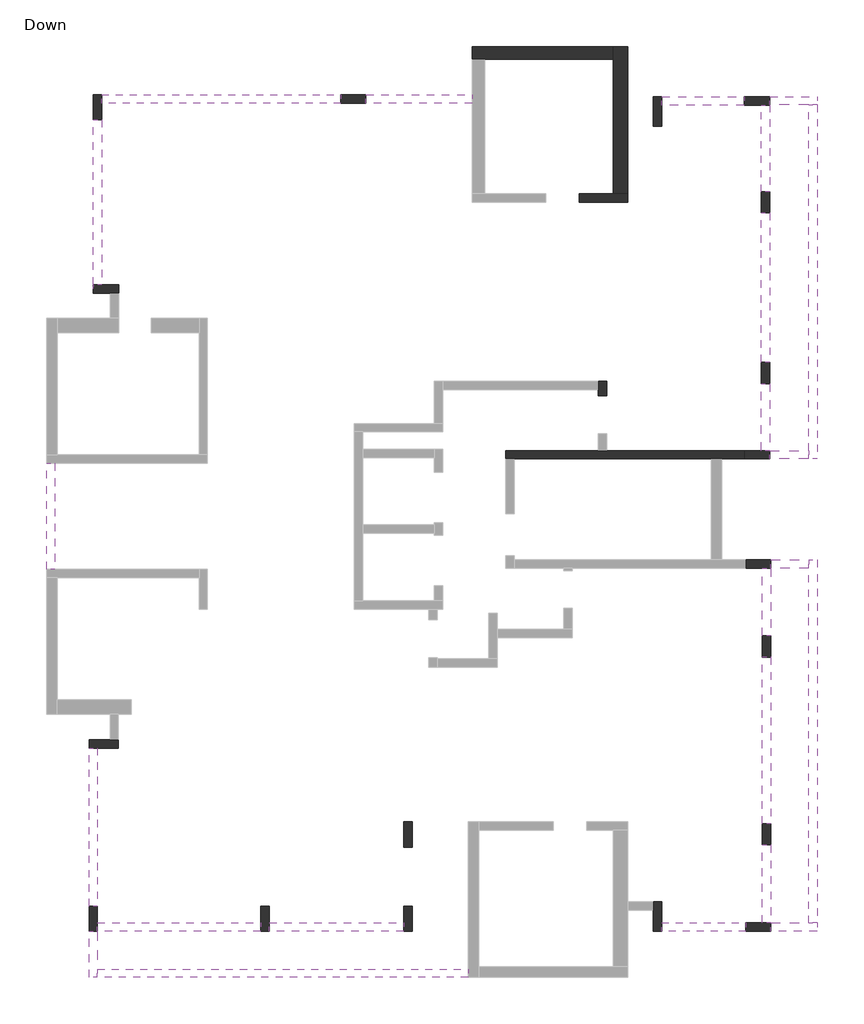
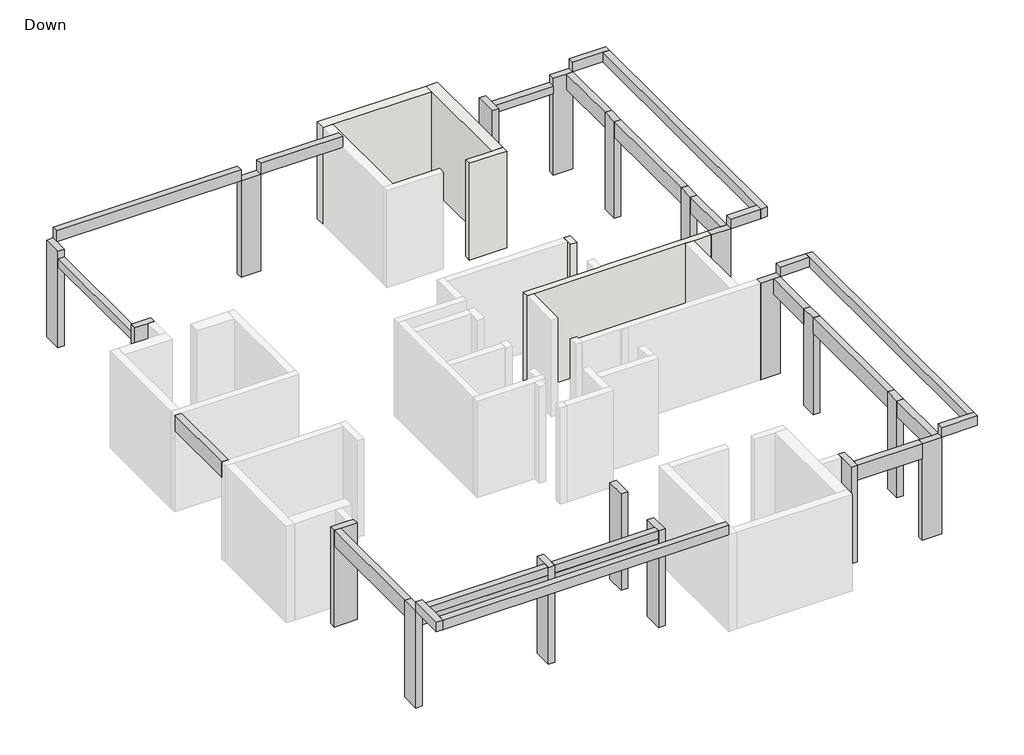
# One storey, part 2 of 2: 23 beams, 18 columns, 5 walls.
"""IFC4 building model written with IfcOpenShell, lengths in millimetres."""

from ifc_helpers import new_model, si_unit, frame, origin, origin_with_axes, place, context, project, spatial, polyline, outline, extrude, faceted_brep, element, save

model = new_model("IFC4")

# Units and contexts
model_context = context("Model", 3, world=origin())
ifc_project = project(units=[si_unit("LENGTHUNIT", "METRE", prefix="MILLI")], contexts=[model_context])

# Site, building, storey
site = spatial("IfcSite", under=ifc_project)
building = spatial("IfcBuilding", under=site)
storey = spatial("IfcBuildingStorey", under=building, Name="Down", Elevation=0.0)

# Beams
placement = place(None, origin())
element("IfcBeam", 1, ObjectType="Concrete Rectengular Beam : 20/50", at=placement, inside=storey, context=model_context, shape_type="Brep", body=[
    faceted_brep([(-11667.5737279, -2465.8036059, 3150.0), (-11467.5737279, -2465.8036059, 3150.0), (-11467.5737279, 47.4292682, 3150.0), (-11667.5737279, 47.4292682, 3150.0), (-11467.5737279, -2465.8036059, 2900.0), (-11467.5737279, -2465.8036059, 2650.0), (-11467.5737279, 47.4292682, 2650.0), (-11467.5737279, 47.4292682, 2900.0), (-11667.5737279, -2465.8036059, 2650.0), (-11667.5737279, 47.4292682, 2650.0)], [[[0, 1, 2, 3]], [[1, 4, 5, 6, 7, 2]], [[5, 8, 9, 6]], [[8, 0, 3, 9]], [[1, 0, 8, 5, 4]], [[3, 2, 7, 6, 9]]]),
])
element("IfcBeam", 2, ObjectType="Concrete Rectengular Beam : 20/50", at=placement, inside=storey, context=model_context, shape_type="Brep", body=[
    faceted_brep([(-10555.9922124, 4197.8205808, 3150.0), (-10555.8228668, 4197.8205808, 3150.0), (-10555.8228668, 4297.8205808, 3150.0), (-10555.9922124, 4297.8205808, 3150.0), (-10355.9922124, 4297.8205808, 2650.0), (-10355.9922124, 8213.0435047, 2650.0), (-10355.9922124, 8213.0435047, 2900.0), (-10355.9922124, 4297.8205808, 2900.0), (-10555.8228668, 4197.8205808, 2650.0), (-10555.9922124, 4197.8205808, 2650.0), (-10555.9922124, 8213.0435047, 2650.0), (-10555.8228668, 4297.8205808, 2650.0), (-10555.9922124, 4297.8205808, 2900.0), (-10555.9922124, 8213.0435047, 2900.0), (-10555.8228668, 4297.8205808, 2900.0)], [[[0, 1, 2, 3]], [[4, 5, 6, 7]], [[8, 9, 10, 5, 4, 11]], [[9, 0, 3, 12, 13, 10]], [[0, 9, 8, 1]], [[11, 4, 7, 14]], [[2, 1, 8, 11, 14]], [[5, 10, 13, 6]], [[12, 14, 7, 6, 13]], [[14, 12, 3, 2]]]),
])
element("IfcBeam", 3, ObjectType="Concrete Rectengular Beam : 20/50", at=placement, inside=storey, context=model_context, shape_type="SweptSolid", body=[
    extrude(outline(polyline([(-1546.8886915, 8813.0435047), (-1546.8886915, 8613.0435047), (-4073.6985753, 8613.0435047), (-4073.6985753, 8813.0435047), (-1546.8886915, 8813.0435047)])), frame((0.0, 0.0, 3150.0), z_axis=(0.0, 0.0, 1.0), x_axis=(1.0, 0.0, 0.0)), (0.0, 0.0, 1.0), 350.0),
])
element("IfcBeam", 4, ObjectType="Concrete Rectengular Beam : 20/50", at=placement, inside=storey, context=model_context, shape_type="SweptSolid", body=[
    extrude(outline(polyline([(2953.3437999, 8567.4646681), (2953.3437999, 8767.4646681), (4922.8790959, 8767.4646681), (4922.8790959, 8567.4646681), (2953.3437999, 8567.4646681)])), frame((0.0, 0.0, 2650.0), z_axis=(0.0, 0.0, 1.0), x_axis=(1.0, 0.0, 0.0)), (0.0, 0.0, 1.0), 250.0),
])
element("IfcBeam", 5, ObjectType="Concrete Rectengular Beam : 20/50", at=placement, inside=storey, context=model_context, shape_type="Brep", body=[
    faceted_brep([(5522.8790959, 8567.4646681, 3150.0), (5322.8790959, 8567.4646681, 3150.0), (5322.8790959, 6503.9942904, 3150.0), (5522.8790959, 6503.9942904, 3150.0), (5522.8790959, 8567.4646681, 2650.0), (5522.8790959, 6503.9942904, 2650.0), (5322.8790959, 8567.4646681, 2650.0), (5322.8790959, 6503.9942904, 2650.0), (5322.8790959, 8567.4646681, 2900.0)], [[[0, 1, 2, 3]], [[4, 0, 3, 5]], [[6, 4, 5, 7]], [[1, 8, 6, 7, 2]], [[1, 0, 4, 6, 8]], [[3, 2, 7, 5]]]),
])
element("IfcBeam", 6, ObjectType="Concrete Rectengular Beam : 20/50", at=placement, inside=storey, context=model_context, shape_type="SweptSolid", body=[
    extrude(outline(polyline([(5322.8790959, 6003.9942904), (5522.8790959, 6003.9942904), (5522.8790959, 2446.2717251), (5322.8790959, 2446.2717251), (5322.8790959, 6003.9942904)])), frame((0.0, 0.0, 2650.0), z_axis=(0.0, 0.0, 1.0), x_axis=(1.0, 0.0, 0.0)), (0.0, 0.0, 1.0), 500.0),
])
element("IfcBeam", 7, ObjectType="Concrete Rectengular Beam : 20/50", at=placement, inside=storey, context=model_context, shape_type="Brep", body=[
    faceted_brep([(5522.8790959, 1946.2717251, 3150.0), (5322.8790959, 1946.2717251, 3150.0), (5322.8790959, 352.3201981, 3150.0), (5522.8790959, 352.3201981, 3150.0), (5322.8790959, 1946.2717251, 2650.0), (5322.8790959, 352.3201981, 2650.0), (5322.8790959, 352.3201981, 2900.0), (5522.8790959, 1946.2717251, 2650.0), (5522.8790959, 352.3201981, 2650.0)], [[[0, 1, 2, 3]], [[1, 4, 5, 6, 2]], [[4, 7, 8, 5]], [[7, 0, 3, 8]], [[1, 0, 7, 4]], [[3, 2, 6, 5, 8]]]),
])
element("IfcBeam", 8, ObjectType="Concrete Rectengular Beam : 20/50", at=placement, inside=storey, context=model_context, shape_type="Brep", body=[
    faceted_brep([(5351.7310336, -4055.4465944, 3150.0), (5551.7310336, -4055.4465944, 3150.0), (5551.7310336, -2446.7479228, 3150.0), (5351.7310336, -2446.7479228, 3150.0), (5351.7310336, -4055.4465944, 2650.0), (5351.7310336, -2446.7479228, 2900.0), (5351.7310336, -2446.7479228, 2650.0), (5551.7310336, -4055.4465944, 2650.0), (5551.7310336, -2446.7479228, 2650.0)], [[[0, 1, 2, 3]], [[4, 0, 3, 5, 6]], [[7, 4, 6, 8]], [[1, 7, 8, 2]], [[1, 0, 4, 7]], [[3, 2, 8, 6, 5]]]),
])
element("IfcBeam", 9, ObjectType="Concrete Rectengular Beam : 20/50", at=placement, inside=storey, context=model_context, shape_type="SweptSolid", body=[
    extrude(outline(polyline([(5551.7310336, -8523.8910533), (5351.7310336, -8523.8910533), (5351.7310336, -4555.4465944), (5551.7310336, -4555.4465944), (5551.7310336, -8523.8910533)])), frame((0.0, 0.0, 2650.0), z_axis=(0.0, 0.0, 1.0), x_axis=(1.0, 0.0, 0.0)), (0.0, 0.0, 1.0), 500.0),
])
element("IfcBeam", 10, ObjectType="Concrete Rectengular Beam : 20/50", at=placement, inside=storey, context=model_context, shape_type="Brep", body=[
    faceted_brep([(5351.7310336, -10874.7377812, 3150.0), (5551.7310336, -10874.7377812, 3150.0), (5551.7310336, -9023.8910533, 3150.0), (5351.7310336, -9023.8910533, 3150.0), (5351.7310336, -10874.7377812, 2650.0), (5351.7310336, -10874.7377812, 2900.0), (5351.7310336, -9023.8910533, 2650.0), (5551.7310336, -10874.7377812, 2650.0), (5551.7310336, -9023.8910533, 2650.0)], [[[0, 1, 2, 3]], [[4, 5, 0, 3, 6]], [[7, 4, 6, 8]], [[1, 7, 8, 2]], [[1, 0, 5, 4, 7]], [[3, 2, 8, 6]]]),
])
element("IfcBeam", 11, ObjectType="Concrete Rectengular Beam : 20/50", at=placement, inside=storey, context=model_context, shape_type="Brep", body=[
    faceted_brep([(2953.3437999, -10874.7377812, 3150.0), (2953.3437999, -11074.7377812, 3150.0), (4951.7310336, -11074.7377812, 3150.0), (4951.7310336, -10874.7377812, 3150.0), (4951.7310336, -10874.7377812, 2900.0), (4951.7310336, -10874.7377812, 2650.0), (2953.3437999, -10874.7377812, 2650.0), (2953.3437999, -10874.7377812, 2900.0), (2953.3437999, -11074.7377812, 2650.0), (4951.7310336, -11074.7377812, 2650.0)], [[[0, 1, 2, 3]], [[0, 3, 4, 5, 6, 7]], [[8, 6, 5, 9]], [[1, 8, 9, 2]], [[1, 0, 7, 6, 8]], [[3, 2, 9, 5, 4]]]),
])
element("IfcBeam", 12, ObjectType="Concrete Rectengular Beam : 20/50", at=placement, inside=storey, context=model_context, shape_type="Brep", body=[
    faceted_brep([(-6576.4457141, -10874.7377812, 3150.0), (-10457.6225223, -10874.7377812, 3150.0), (-10457.6225223, -11073.8349319, 3150.0), (-6576.4457141, -11073.8349319, 3150.0), (-10457.6225223, -10874.7377812, 2650.0), (-10457.6225223, -10874.7377812, 2900.0), (-6576.4457141, -10874.7377812, 2900.0), (-6576.4457141, -10874.7377812, 2650.0), (-10457.6225223, -11074.7377812, 2650.0), (-6576.4457141, -11074.7377812, 2650.0), (-6576.4457141, -11074.7377812, 2900.0), (-10457.6225223, -11074.7377812, 2900.0), (-10457.6225223, -11073.8349319, 2900.0), (-6576.4457141, -11073.8349319, 2900.0)], [[[0, 1, 2, 3]], [[4, 5, 1, 0, 6, 7]], [[8, 4, 7, 9]], [[8, 9, 10, 11]], [[4, 8, 11, 12, 2, 1, 5]], [[9, 7, 6, 0, 3, 13, 10]], [[13, 12, 11, 10]], [[12, 13, 3, 2]]]),
])
element("IfcBeam", 13, ObjectType="Concrete Rectengular Beam : 20/50", at=placement, inside=storey, context=model_context, shape_type="Brep", body=[
    faceted_brep([(-10657.6225223, -10475.5031849, 3150.0), (-10457.6225223, -10475.5031849, 3150.0), (-10457.6225223, -6721.9995493, 3150.0), (-10657.6225223, -6721.9995493, 3150.0), (-10457.6225223, -10475.5031849, 2900.0), (-10457.6225223, -10475.5031849, 2650.0), (-10457.6225223, -6721.9995493, 2650.0), (-10457.6225223, -6721.9995493, 2900.0), (-10657.6225223, -10475.5031849, 2650.0), (-10657.6225223, -6721.9995493, 2650.0)], [[[0, 1, 2, 3]], [[2, 1, 4, 5, 6, 7]], [[5, 8, 9, 6]], [[8, 0, 3, 9]], [[1, 0, 8, 5, 4]], [[3, 2, 7, 6, 9]]]),
])
element("IfcBeam", 14, ObjectType="Concrete Rectengular Beam : 20/50", at=placement, inside=storey, context=model_context, shape_type="Brep", body=[
    faceted_brep([(-3172.9736513, -10874.7377812, 3150.0), (-6376.4457141, -10874.7377812, 3150.0), (-6376.4457141, -11073.8349319, 3150.0), (-3172.9736513, -11073.8349319, 3150.0), (-6376.4457141, -11074.7377812, 2650.0), (-3172.9736513, -11074.7377812, 2650.0), (-3172.9736513, -11074.7377812, 2900.0), (-6376.4457141, -11074.7377812, 2900.0), (-6376.4457141, -10874.7377812, 2650.0), (-3172.9736513, -10874.7377812, 2650.0), (-3172.9736513, -10874.7377812, 2900.0), (-6376.4457141, -10874.7377812, 2900.0), (-6376.4457141, -11073.8349319, 2900.0), (-3172.9736513, -11073.8349319, 2900.0)], [[[0, 1, 2, 3]], [[4, 5, 6, 7]], [[4, 8, 9, 5]], [[1, 0, 10, 9, 8, 11]], [[8, 4, 7, 12, 2, 1, 11]], [[5, 9, 10, 0, 3, 13, 6]], [[13, 12, 7, 6]], [[12, 13, 3, 2]]]),
])
element("IfcBeam", 15, ObjectType="Concrete Rectengular Beam : 20/56", at=placement, inside=storey, context=model_context, shape_type="Brep", body=[
    faceted_brep([(6650.1463257, 8767.4646681, 3460.0), (5522.8790959, 8767.4646681, 3460.0), (5522.8790959, 8567.4646681, 3460.0), (6450.1463257, 8567.4646681, 3460.0), (6650.1463257, 8567.4646681, 3460.0), (5522.8790959, 8567.4646681, 3150.0), (6450.1463257, 8567.4646681, 3150.0), (6650.1463257, 8567.4646681, 3150.0), (6650.1463257, 8767.4646681, 3150.0), (5522.8790959, 8767.4646681, 3150.0)], [[[0, 1, 2, 3, 4]], [[4, 3, 2, 5, 6, 7]], [[1, 0, 8, 9]], [[0, 4, 7, 8]], [[7, 6, 5, 9, 8]], [[2, 1, 9, 5]]]),
])
element("IfcBeam", 16, ObjectType="Concrete Rectengular Beam : 20/56", at=placement, inside=storey, context=model_context, shape_type="Brep", body=[
    faceted_brep([(6650.1463257, 8567.4646681, 3460.0), (6450.1463257, 8567.4646681, 3460.0), (6450.1463257, 352.3201981, 3460.0), (6450.1463257, 152.3201981, 3460.0), (6650.1463257, 152.3201981, 3460.0), (6450.1463257, 8567.4646681, 3150.0), (6450.1463257, 352.3201981, 3150.0), (6450.1463257, 152.3201981, 3150.0), (6650.1463257, 152.3201981, 3150.0), (6650.1463257, 8567.4646681, 3150.0)], [[[0, 1, 2, 3, 4]], [[3, 2, 1, 5, 6, 7]], [[0, 4, 8, 9]], [[1, 0, 9, 5]], [[4, 3, 7, 8]], [[7, 6, 5, 9, 8]]]),
])
element("IfcBeam", 17, ObjectType="Concrete Rectengular Beam : 20/56", at=placement, inside=storey, context=model_context, shape_type="SweptSolid", body=[
    extrude(outline(polyline([(5522.8790959, 152.3201981), (5522.8790959, 352.3201981), (6450.1463257, 352.3201981), (6450.1463257, 152.3201981), (5522.8790959, 152.3201981)])), frame((0.0, 0.0, 3150.0), z_axis=(0.0, 0.0, 1.0), x_axis=(1.0, 0.0, 0.0)), (0.0, 0.0, 1.0), 310.0),
])
element("IfcBeam", 18, ObjectType="Concrete Rectengular Beam : 20/56", at=placement, inside=storey, context=model_context, shape_type="Brep", body=[
    faceted_brep([(-10657.6225223, -11075.5031849, 3460.0), (-10457.6225223, -11075.5031849, 3460.0), (-10457.6225223, -11075.5031849, 3150.0), (-10657.6225223, -11075.5031849, 3150.0), (-10657.6225223, -12173.6155079, 3460.0), (-10457.6225223, -12173.6155079, 3460.0), (-10457.6225223, -11973.6155079, 3460.0), (-10657.6225223, -12173.6155079, 3150.0), (-10457.6225223, -12173.6155079, 3150.0), (-10457.6225223, -11973.6155079, 3150.0)], [[[0, 1, 2, 3]], [[1, 0, 4, 5, 6]], [[4, 0, 3, 7]], [[1, 6, 5, 8, 9, 2]], [[5, 4, 7, 8]], [[3, 2, 9, 8, 7]]]),
])
element("IfcBeam", 19, ObjectType="Concrete Rectengular Beam : 20/56", at=placement, inside=storey, context=model_context, shape_type="SweptSolid", body=[
    extrude(outline(polyline([(-1646.4017034, -11973.6155079), (-1646.4017034, -12173.6155079), (-10457.6225223, -12173.6155079), (-10457.6225223, -11973.6155079), (-1646.4017034, -11973.6155079)])), frame((0.0, 0.0, 3150.0), z_axis=(0.0, 0.0, 1.0), x_axis=(1.0, 0.0, 0.0)), (0.0, 0.0, 1.0), 310.0),
])
element("IfcBeam", 20, ObjectType="Concrete Rectengular Beam : 20/56", at=placement, inside=storey, context=model_context, shape_type="Brep", body=[
    faceted_brep([(5551.7310336, -11074.7377812, 3460.0), (5551.7310336, -10874.7377812, 3460.0), (5551.7310336, -10874.7377812, 3150.0), (5551.7310336, -11074.7377812, 3150.0), (6650.1463257, -11074.7377812, 3460.0), (6650.1463257, -10874.7377812, 3460.0), (6450.1463257, -10874.7377812, 3460.0), (6650.1463257, -11074.7377812, 3150.0), (6650.1463257, -10874.7377812, 3150.0), (6450.1463257, -10874.7377812, 3150.0)], [[[0, 1, 2, 3]], [[1, 0, 4, 5, 6]], [[4, 0, 3, 7]], [[1, 6, 5, 8, 9, 2]], [[5, 4, 7, 8]], [[3, 2, 9, 8, 7]]]),
])
element("IfcBeam", 21, ObjectType="Concrete Rectengular Beam : 20/56", at=placement, inside=storey, context=model_context, shape_type="Brep", body=[
    faceted_brep([(6650.1463257, -2246.7479228, 3460.0), (6450.1463257, -2246.7479228, 3460.0), (6450.1463257, -2446.7479228, 3460.0), (6450.1463257, -10874.7377812, 3460.0), (6650.1463257, -10874.7377812, 3460.0), (6650.1463257, -10874.7377812, 3150.0), (6650.1463257, -2246.7479228, 3150.0), (6450.1463257, -2246.7479228, 3150.0), (6450.1463257, -2446.7479228, 3150.0), (6450.1463257, -10874.7377812, 3150.0)], [[[0, 1, 2, 3, 4]], [[0, 4, 5, 6]], [[3, 2, 1, 7, 8, 9]], [[4, 3, 9, 5]], [[1, 0, 6, 7]], [[6, 5, 9, 8, 7]]]),
])
element("IfcBeam", 22, ObjectType="Concrete Rectengular Beam : 20/56", at=placement, inside=storey, context=model_context, shape_type="SweptSolid", body=[
    extrude(outline(polyline([(5551.7310336, -2446.7479228), (5551.7310336, -2246.7479228), (6450.1463257, -2246.7479228), (6450.1463257, -2446.7479228), (5551.7310336, -2446.7479228)])), frame((0.0, 0.0, 3150.0), z_axis=(0.0, 0.0, 1.0), x_axis=(1.0, 0.0, 0.0)), (0.0, 0.0, 1.0), 310.0),
])
element("IfcBeam", 23, ObjectType="Concrete Rectengular Beam : 20/60", at=placement, inside=storey, context=model_context, shape_type="SweptSolid", body=[
    extrude(outline(polyline([(-10355.9922124, 8613.0435047), (-10355.9922124, 8813.0435047), (-4673.6985753, 8813.0435047), (-4673.6985753, 8613.0435047), (-10355.9922124, 8613.0435047)])), frame((0.0, 0.0, 3150.0), z_axis=(0.0, 0.0, 1.0), x_axis=(1.0, 0.0, 0.0)), (0.0, 0.0, 1.0), 350.0),
])

# Columns
element("IfcColumn", 24, ObjectType="Concrete Rectengular Column : 20/50", at=placement, inside=storey, context=model_context, shape_type="SweptSolid", body=[
    extrude(outline(polyline([(5551.7310336, -8523.8910533), (5551.7310336, -9023.8910533), (5351.7310336, -9023.8910533), (5351.7310336, -8523.8910533), (5551.7310336, -8523.8910533)])), origin_with_axes(), (0.0, 0.0, 1.0), 3150.0),
])
element("IfcColumn", 25, ObjectType="Concrete Rectengular Column : 20/50", at=placement, inside=storey, context=model_context, shape_type="SweptSolid", body=[
    extrude(outline(polyline([(5551.7310336, -4055.4465944), (5551.7310336, -4555.4465944), (5351.7310336, -4555.4465944), (5351.7310336, -4055.4465944), (5551.7310336, -4055.4465944)])), origin_with_axes(), (0.0, 0.0, 1.0), 3150.0),
])
element("IfcColumn", 26, ObjectType="Concrete Rectengular Column : 20/50", at=placement, inside=storey, context=model_context, shape_type="SweptSolid", body=[
    extrude(outline(polyline([(5522.8790959, 6503.9942904), (5522.8790959, 6003.9942904), (5322.8790959, 6003.9942904), (5322.8790959, 6503.9942904), (5522.8790959, 6503.9942904)])), origin_with_axes(), (0.0, 0.0, 1.0), 3150.0),
])
element("IfcColumn", 27, ObjectType="Concrete Rectengular Column : 20/50", at=placement, inside=storey, context=model_context, shape_type="SweptSolid", body=[
    extrude(outline(polyline([(5522.8790959, 2446.2717251), (5522.8790959, 1946.2717251), (5322.8790959, 1946.2717251), (5322.8790959, 2446.2717251), (5522.8790959, 2446.2717251)])), origin_with_axes(), (0.0, 0.0, 1.0), 3150.0),
])
element("IfcColumn", 28, ObjectType="Concrete Rectengular Column : 20/60", at=placement, inside=storey, context=model_context, shape_type="Brep", body=[
    faceted_brep([(-10457.6225223, -10475.5031849, 0.0), (-10457.6225223, -11075.5031849, 0.0), (-10657.6225223, -11075.5031849, 0.0), (-10657.6225223, -10475.5031849, 0.0), (-10457.6225223, -10475.5031849, 3150.0), (-10457.6225223, -10874.7377812, 3150.0), (-10457.6225223, -11073.8349319, 3150.0), (-10457.6225223, -11075.5031849, 3150.0), (-10457.6225223, -11075.5031849, 2900.0), (-10657.6225223, -11075.5031849, 3150.0), (-10657.6225223, -11075.5031849, 2900.0), (-10657.6225223, -10475.5031849, 3150.0)], [[[0, 1, 2, 3]], [[4, 5, 6, 7, 8, 1, 0]], [[7, 9, 10, 2, 1, 8]], [[9, 11, 3, 2, 10]], [[11, 4, 0, 3]], [[4, 11, 9, 7, 6, 5]]]),
])
element("IfcColumn", 29, ObjectType="Concrete Rectengular Column : 20/60", at=placement, inside=storey, context=model_context, shape_type="Brep", body=[
    faceted_brep([(-6376.4457141, -10475.5031849, 0.0), (-6376.4457141, -11075.5031849, 0.0), (-6576.4457141, -11075.5031849, 0.0), (-6576.4457141, -10475.5031849, 0.0), (-6376.4457141, -10475.5031849, 3150.0), (-6376.4457141, -10874.7377812, 3150.0), (-6376.4457141, -11073.8349319, 3150.0), (-6376.4457141, -11075.5031849, 3150.0), (-6376.4457141, -11075.5031849, 2900.0), (-6376.4457141, -10475.5031849, 2900.0), (-6576.4457141, -11075.5031849, 3150.0), (-6576.4457141, -11075.5031849, 2900.0), (-6576.4457141, -11073.8349319, 3150.0), (-6576.4457141, -10874.7377812, 3150.0), (-6576.4457141, -10475.5031849, 3150.0), (-6576.4457141, -10475.5031849, 2900.0)], [[[0, 1, 2, 3]], [[4, 5, 6, 7, 8, 1, 0, 9]], [[7, 10, 11, 2, 1, 8]], [[10, 12, 13, 14, 15, 3, 2, 11]], [[14, 4, 9, 0, 3, 15]], [[4, 14, 13, 12, 10, 7, 6, 5]]]),
])
element("IfcColumn", 30, ObjectType="Concrete Rectengular Column : 20/60", at=placement, inside=storey, context=model_context, shape_type="Brep", body=[
    faceted_brep([(-2972.9736513, -10475.5031849, 0.0), (-2972.9736513, -11075.5031849, 0.0), (-3172.9736513, -11075.5031849, 0.0), (-3172.9736513, -10475.5031849, 0.0), (-2972.9736513, -10475.5031849, 3150.0), (-2972.9736513, -11075.5031849, 3150.0), (-2972.9736513, -11075.5031849, 2900.0), (-3172.9736513, -11075.5031849, 3150.0), (-3172.9736513, -11075.5031849, 2900.0), (-3172.9736513, -11073.8349319, 3150.0), (-3172.9736513, -10874.7377812, 3150.0), (-3172.9736513, -10475.5031849, 3150.0)], [[[0, 1, 2, 3]], [[4, 5, 6, 1, 0]], [[5, 7, 8, 2, 1, 6]], [[7, 9, 10, 11, 3, 2, 8]], [[11, 4, 0, 3]], [[4, 11, 10, 9, 7, 5]]]),
])
element("IfcColumn", 31, ObjectType="Concrete Rectengular Column : 20/60", at=placement, inside=storey, context=model_context, shape_type="Brep", body=[
    faceted_brep([(-2972.9736513, -8473.8910533, 0.0), (-2972.9736513, -9073.8910533, 0.0), (-3172.9736513, -9073.8910533, 0.0), (-3172.9736513, -8473.8910533, 0.0), (-2972.9736513, -8473.8910533, 3150.0), (-2972.9736513, -9073.8910533, 3150.0), (-2972.9736513, -8473.8910533, 2900.0), (-3172.9736513, -9073.8910533, 3150.0), (-3172.9736513, -8473.8910533, 3150.0), (-3172.9736513, -8473.8910533, 2900.0)], [[[0, 1, 2, 3]], [[4, 5, 1, 0, 6]], [[5, 7, 2, 1]], [[7, 8, 9, 3, 2]], [[8, 4, 6, 0, 3, 9]], [[4, 8, 7, 5]]]),
])
element("IfcColumn", 32, ObjectType="Concrete Rectengular Column : 20/60", at=placement, inside=storey, context=model_context, shape_type="Brep", body=[
    faceted_brep([(-10555.8228668, 4297.8205808, 0.0), (-9955.8228668, 4297.8205808, 0.0), (-9955.8228668, 4097.8205808, 0.0), (-10155.8228668, 4097.8205808, 0.0), (-10555.8228668, 4097.8205808, 0.0), (-10555.8228668, 4297.8205808, 3150.0), (-9955.8228668, 4297.8205808, 3150.0), (-9955.8228668, 4297.8205808, 2900.0), (-9955.8228668, 4097.8205808, 3150.0), (-10155.8228668, 4097.8205808, 3150.0), (-10555.8228668, 4097.8205808, 3150.0)], [[[0, 1, 2, 3, 4]], [[5, 6, 7, 1, 0]], [[6, 8, 2, 1, 7]], [[8, 9, 10, 4, 3, 2]], [[10, 5, 0, 4]], [[5, 10, 9, 8, 6]]]),
])
element("IfcColumn", 33, ObjectType="Concrete Rectengular Column : 20/60", at=placement, inside=storey, context=model_context, shape_type="Brep", body=[
    faceted_brep([(-10555.9922124, 8213.0435047, 0.0), (-10555.9922124, 8813.0435047, 0.0), (-10355.9922124, 8813.0435047, 0.0), (-10355.9922124, 8213.0435047, 0.0), (-10555.9922124, 8213.0435047, 3150.0), (-10555.9922124, 8813.0435047, 3150.0), (-10555.9922124, 8213.0435047, 2900.0), (-10355.9922124, 8813.0435047, 3150.0), (-10355.9922124, 8813.0435047, 2900.0), (-10355.9922124, 8213.0435047, 3150.0), (-10355.9922124, 8213.0435047, 2900.0)], [[[0, 1, 2, 3]], [[4, 5, 1, 0, 6]], [[5, 7, 8, 2, 1]], [[7, 9, 10, 3, 2, 8]], [[9, 4, 6, 0, 3, 10]], [[4, 9, 7, 5]]]),
])
element("IfcColumn", 34, ObjectType="Concrete Rectengular Column : 20/60", at=placement, inside=storey, context=model_context, shape_type="Brep", body=[
    faceted_brep([(-4673.6985753, 8813.0435047, 0.0), (-4073.6985753, 8813.0435047, 0.0), (-4073.6985753, 8613.0435047, 0.0), (-4673.6985753, 8613.0435047, 0.0), (-4673.6985753, 8813.0435047, 3150.0), (-4073.6985753, 8813.0435047, 3150.0), (-4073.6985753, 8813.0435047, 2900.0), (-4673.6985753, 8813.0435047, 2900.0), (-4073.6985753, 8613.0435047, 3150.0), (-4073.6985753, 8613.0435047, 2900.0), (-4673.6985753, 8613.0435047, 3150.0), (-4673.6985753, 8613.0435047, 2900.0)], [[[0, 1, 2, 3]], [[4, 5, 6, 1, 0, 7]], [[5, 8, 9, 2, 1, 6]], [[8, 10, 11, 3, 2, 9]], [[10, 4, 7, 0, 3, 11]], [[4, 10, 8, 5]]]),
])
element("IfcColumn", 35, ObjectType="Concrete Rectengular Column : 20/60", at=placement, inside=storey, context=model_context, shape_type="Brep", body=[
    faceted_brep([(4951.7310336, -10874.7377812, 0.0), (5551.7310336, -10874.7377812, 0.0), (5551.7310336, -11074.7377812, 0.0), (4951.7310336, -11074.7377812, 0.0), (4951.7310336, -10874.7377812, 3150.0), (5351.7310336, -10874.7377812, 3150.0), (5551.7310336, -10874.7377812, 3150.0), (5551.7310336, -11074.7377812, 3150.0), (5551.7310336, -11074.7377812, 2900.0), (4951.7310336, -11074.7377812, 3150.0)], [[[0, 1, 2, 3]], [[4, 5, 6, 1, 0]], [[6, 7, 8, 2, 1]], [[7, 9, 3, 2, 8]], [[9, 4, 0, 3]], [[4, 9, 7, 6, 5]]]),
])
element("IfcColumn", 36, ObjectType="Concrete Rectengular Column : 20/60", at=placement, inside=storey, context=model_context, shape_type="Brep", body=[
    faceted_brep([(4951.7310336, -2246.7479228, 0.0), (5551.7310336, -2246.7479228, 0.0), (5551.7310336, -2446.7479228, 0.0), (4951.7310336, -2446.7479228, 0.0), (4951.7310336, -2246.7479228, 3150.0), (5551.7310336, -2246.7479228, 3150.0), (5551.7310336, -2246.7479228, 2900.0), (5551.7310336, -2446.7479228, 3150.0), (5351.7310336, -2446.7479228, 3150.0), (4951.7310336, -2446.7479228, 3150.0)], [[[0, 1, 2, 3]], [[4, 5, 6, 1, 0]], [[5, 7, 2, 1, 6]], [[7, 8, 9, 3, 2]], [[9, 4, 0, 3]], [[4, 9, 8, 7, 5]]]),
])
element("IfcColumn", 37, ObjectType="Concrete Rectengular Column : 20/60", at=placement, inside=storey, context=model_context, shape_type="Brep", body=[
    faceted_brep([(4922.8790959, 8767.4646681, 0.0), (5522.8790959, 8767.4646681, 0.0), (5522.8790959, 8567.4646681, 0.0), (4922.8790959, 8567.4646681, 0.0), (4922.8790959, 8767.4646681, 3150.0), (5522.8790959, 8767.4646681, 3150.0), (5522.8790959, 8767.4646681, 2900.0), (4922.8790959, 8767.4646681, 2900.0), (5522.8790959, 8567.4646681, 3150.0), (5322.8790959, 8567.4646681, 3150.0), (4922.8790959, 8567.4646681, 3150.0), (4922.8790959, 8567.4646681, 2900.0)], [[[0, 1, 2, 3]], [[4, 5, 6, 1, 0, 7]], [[5, 8, 2, 1, 6]], [[8, 9, 10, 11, 3, 2]], [[10, 4, 7, 0, 3, 11]], [[4, 10, 9, 8, 5]]]),
])
element("IfcColumn", 38, ObjectType="Concrete Rectengular Column : 20/60", at=placement, inside=storey, context=model_context, shape_type="Brep", body=[
    faceted_brep([(4922.8790959, 352.3201981, 0.0), (5522.8790959, 352.3201981, 0.0), (5522.8790959, 152.3201981, 0.0), (4922.8790959, 152.3201981, 0.0), (4922.8790959, 352.3201981, 3150.0), (5322.8790959, 352.3201981, 3150.0), (5522.8790959, 352.3201981, 3150.0), (5522.8790959, 152.3201981, 3150.0), (5522.8790959, 152.3201981, 2900.0), (4922.8790959, 152.3201981, 3150.0)], [[[0, 1, 2, 3]], [[4, 5, 6, 1, 0]], [[6, 7, 8, 2, 1]], [[7, 9, 3, 2, 8]], [[9, 4, 0, 3]], [[4, 9, 7, 6, 5]]]),
])
element("IfcColumn", 39, ObjectType="Concrete Rectengular Column : 20/70", at=placement, inside=storey, context=model_context, shape_type="Brep", body=[
    faceted_brep([(-10657.6225223, -6521.9995493, 0.0), (-10157.6225223, -6521.9995493, 0.0), (-9957.6225223, -6521.9995493, 0.0), (-9957.6225223, -6721.9995493, 0.0), (-10657.6225223, -6721.9995493, 0.0), (-10657.6225223, -6521.9995493, 3150.0), (-10157.6225223, -6521.9995493, 3150.0), (-9957.6225223, -6521.9995493, 3150.0), (-9957.6225223, -6721.9995493, 3150.0), (-9957.6225223, -6721.9995493, 2900.0), (-10457.6225223, -6721.9995493, 3150.0), (-10657.6225223, -6721.9995493, 3150.0), (-10657.6225223, -6721.9995493, 2650.0)], [[[0, 1, 2, 3, 4]], [[5, 6, 7, 2, 1, 0]], [[7, 8, 9, 3, 2]], [[8, 10, 11, 12, 4, 3, 9]], [[11, 5, 0, 4, 12]], [[5, 11, 10, 8, 7, 6]]]),
])
element("IfcColumn", 40, ObjectType="Concrete Rectengular Column : 20/70", at=placement, inside=storey, context=model_context, shape_type="Brep", body=[
    faceted_brep([(2953.3437999, -10374.7377812, 0.0), (2953.3437999, -11074.7377812, 0.0), (2753.3437999, -11074.7377812, 0.0), (2753.3437999, -10574.7377812, 0.0), (2753.3437999, -10374.7377812, 0.0), (2953.3437999, -10374.7377812, 3150.0), (2953.3437999, -10874.7377812, 3150.0), (2953.3437999, -11074.7377812, 3150.0), (2953.3437999, -10374.7377812, 2900.0), (2753.3437999, -11074.7377812, 3150.0), (2753.3437999, -10574.7377812, 3150.0), (2753.3437999, -10374.7377812, 3150.0)], [[[0, 1, 2, 3, 4]], [[5, 6, 7, 1, 0, 8]], [[7, 9, 2, 1]], [[9, 10, 11, 4, 3, 2]], [[11, 5, 8, 0, 4]], [[5, 11, 10, 9, 7, 6]]]),
])
element("IfcColumn", 41, ObjectType="Concrete Rectengular Column : 20/70", at=placement, inside=storey, context=model_context, shape_type="Brep", body=[
    faceted_brep([(2953.3437999, 8767.4646681, 0.0), (2953.3437999, 8067.4646681, 0.0), (2753.3437999, 8067.4646681, 0.0), (2753.3437999, 8767.4646681, 0.0), (2953.3437999, 8767.4646681, 3150.0), (2953.3437999, 8067.4646681, 3150.0), (2953.3437999, 8067.4646681, 2900.0), (2953.3437999, 8767.4646681, 2900.0), (2753.3437999, 8067.4646681, 3150.0), (2753.3437999, 8767.4646681, 3150.0)], [[[0, 1, 2, 3]], [[4, 5, 6, 1, 0, 7]], [[5, 8, 2, 1, 6]], [[8, 9, 3, 2]], [[9, 4, 7, 0, 3]], [[4, 9, 8, 5]]]),
])

# Walls
element("IfcWall", 42, ObjectType="20", at=placement, inside=storey, context=model_context, shape_type="Brep", body=[
    faceted_brep([(1452.348775, 2003.8127355, 0.0), (1452.348775, 1803.8127355, 0.0), (1452.348775, 1652.3412467, 0.0), (1452.348775, 1652.3412467, 2900.0), (1452.348775, 1652.3412467, 3150.0), (1452.348775, 1803.8127355, 3150.0), (1452.348775, 2003.8127355, 3150.0), (1652.348775, 2003.8127355, 0.0), (1652.348775, 2003.8127355, 2900.0), (1652.348775, 2003.8127355, 3150.0), (1652.348775, 1652.3412467, 3150.0), (1652.348775, 1652.3412467, 2900.0), (1652.348775, 1652.3412467, 0.0), (1552.348775, 1652.3412467, 3150.0)], [[[0, 1, 2, 3, 4, 5, 6]], [[7, 8, 9, 10, 11, 12]], [[2, 1, 0, 7, 12]], [[4, 3, 2, 12, 11, 10, 13]], [[6, 5, 4, 13, 10, 9]], [[0, 6, 9, 8, 7]]]),
])
element("IfcWall", 43, ObjectType="20", at=placement, inside=storey, context=model_context, shape_type="Brep", body=[
    faceted_brep([(-748.6672985, 152.3201981, 0.0), (-548.6672985, 152.3201981, 0.0), (4133.663356, 152.3201981, 0.0), (4383.663356, 152.3201981, 0.0), (4922.8790959, 152.3201981, 0.0), (4922.8790959, 152.3201981, 3150.0), (4383.663356, 152.3201981, 3150.0), (4133.663356, 152.3201981, 3150.0), (-548.6672985, 152.3201981, 3150.0), (-748.6672985, 152.3201981, 3150.0), (-748.6672985, 352.3201981, 0.0), (-748.6672985, 352.3201981, 2900.0), (-748.6672985, 352.3201981, 3150.0), (1452.348775, 352.3201981, 3150.0), (1652.348775, 352.3201981, 3150.0), (4922.8790959, 352.3201981, 3150.0), (4922.8790959, 352.3201981, 0.0), (1652.348775, 352.3201981, 0.0), (1452.348775, 352.3201981, 0.0)], [[[0, 1, 2, 3, 4, 5, 6, 7, 8, 9]], [[10, 11, 12, 13, 14, 15, 16, 17, 18]], [[4, 3, 2, 1, 0, 10, 18, 17, 16]], [[5, 4, 16, 15]], [[9, 8, 7, 6, 5, 15, 14, 13, 12]], [[0, 9, 12, 11, 10]]]),
])
element("IfcWall", 44, ObjectType="20", at=placement, inside=storey, context=model_context, shape_type="Brep", body=[
    faceted_brep([(1000.2209526, 6257.4646681, 0.0), (2149.9138343, 6257.4646681, 0.0), (2149.9138343, 6257.4646681, 2900.0), (2149.9138343, 6257.4646681, 3150.0), (1000.2209526, 6257.4646681, 3150.0), (1000.2209526, 6257.4646681, 2900.0), (1000.2209526, 6457.4646681, 0.0), (1000.2209526, 6457.4646681, 2900.0), (1000.2209526, 6457.4646681, 3150.0), (1799.9138343, 6457.4646681, 3150.0), (2149.9138343, 6457.4646681, 3150.0), (2149.9138343, 6457.4646681, 0.0), (1799.9138343, 6457.4646681, 0.0)], [[[0, 1, 2, 3, 4, 5]], [[6, 7, 8, 9, 10, 11, 12]], [[1, 0, 6, 12, 11]], [[4, 3, 10, 9, 8]], [[0, 5, 4, 8, 7, 6]], [[3, 2, 1, 11, 10]]]),
])
element("IfcWall", 45, ObjectType="30", at=placement, inside=storey, context=model_context, shape_type="Brep", body=[
    faceted_brep([(1799.9138343, 9957.4646681, 0.0), (-1546.8886915, 9957.4646681, 0.0), (-1546.8886915, 9957.4646681, 3150.0), (1799.9138343, 9957.4646681, 3150.0), (1799.9138343, 9657.4646681, 0.0), (1799.9138343, 9657.4646681, 2900.0), (1799.9138343, 9657.4646681, 3150.0), (-1246.8886915, 9657.4646681, 3150.0), (-1546.8886915, 9657.4646681, 3150.0), (-1546.8886915, 9657.4646681, 0.0), (-1246.8886915, 9657.4646681, 0.0)], [[[0, 1, 2, 3]], [[4, 5, 6, 7, 8, 9, 10]], [[1, 0, 4, 10, 9]], [[3, 2, 8, 7, 6]], [[0, 3, 6, 5, 4]], [[2, 1, 9, 8]]]),
])
element("IfcWall", 46, ObjectType="35", at=placement, inside=storey, context=model_context, shape_type="Brep", body=[
    faceted_brep([(2149.9138343, 6457.4646681, 0.0), (2149.9138343, 9957.4646681, 0.0), (2149.9138343, 9957.4646681, 3150.0), (2149.9138343, 8067.4646681, 3150.0), (2149.9138343, 6457.4646681, 3150.0), (1799.9138343, 6457.4646681, 0.0), (1799.9138343, 6457.4646681, 2900.0), (1799.9138343, 6457.4646681, 3150.0), (1799.9138343, 9657.4646681, 3150.0), (1799.9138343, 9957.4646681, 3150.0), (1799.9138343, 9957.4646681, 0.0), (1799.9138343, 9657.4646681, 0.0)], [[[0, 1, 2, 3, 4]], [[5, 6, 7, 8, 9, 10, 11]], [[1, 0, 5, 11, 10]], [[4, 3, 2, 9, 8, 7]], [[0, 4, 7, 6, 5]], [[2, 1, 10, 9]]]),
])

save(model, "model.ifc")

# Revit data of these elements
# Type "Concrete Rectengular Beam : 20/50"
#   Length [instance default] = 152.4 cm
#   b = 20 cm
#   h = 50 cm
#   Structural Material [instance default] = Concrete
#   Assembly Code = ""
# Type "Concrete Rectengular Beam : 20/56"
#   Length [instance default] = 152.4 cm
#   b = 20 cm
#   h = 56 cm
#   Structural Material [instance default] = Concrete
#   Assembly Code = ""
# Type "Concrete Rectengular Beam : 20/60"
#   Length [instance default] = 152.4 cm
#   b = 20 cm
#   h = 60 cm
#   Structural Material [instance default] = Concrete
#   Assembly Code = ""
# Type "Concrete Rectengular Column : 20/50"
#   b = 20 cm
#   h = 50 cm
#   Structural Material [instance default] = Concrete
# Type "Concrete Rectengular Column : 20/60"
#   b = 20 cm
#   h = 60 cm
#   Structural Material [instance default] = Concrete
# Type "Concrete Rectengular Column : 20/70"
#   b = 20 cm
#   h = 70 cm
#   Structural Material [instance default] = Concrete
# Type "20"
#   Layers, outside or top first: 20 cm "Concrete" (function 1)
# Type "30"
#   Layers, outside or top first: 30 cm "Concrete" (function 1)
# Type "35"
#   Layers, outside or top first: 35 cm "Concrete" (function 1)
# Element 1 (IfcBeam, "Concrete Rectengular Beam : 20/50")
#   Comments = ""
#   Mark = "B2"
#   SOFiSTiK_AMG_Comments = ""
#   SOFiSTiK_AMG_Scheduled = yes
#   SOFiSTiK_AMG_Adjusted = yes
#   Structural Material = Concrete
#   Phase Created = New Construction
#   Materials on its faces: "Concrete"
# Element 2 (IfcBeam, "Concrete Rectengular Beam : 20/50")
#   Comments = ""
#   Mark = "B3"
#   SOFiSTiK_AMG_Comments = ""
#   SOFiSTiK_AMG_Scheduled = yes
#   SOFiSTiK_AMG_Adjusted = yes
#   Structural Material = Concrete
#   Phase Created = New Construction
#   Materials on its faces: "Concrete"
# Element 3 (IfcBeam, "Concrete Rectengular Beam : 20/50")
#   Comments = ""
#   Mark = "B4"
#   SOFiSTiK_AMG_Comments = ""
#   SOFiSTiK_AMG_Scheduled = yes
#   SOFiSTiK_AMG_Adjusted = yes
#   Structural Material = Concrete
#   Phase Created = New Construction
#   Materials on its faces: "Concrete"
# Element 4 (IfcBeam, "Concrete Rectengular Beam : 20/50")
#   Comments = ""
#   Mark = "B5"
#   SOFiSTiK_AMG_Comments = ""
#   SOFiSTiK_AMG_Scheduled = yes
#   SOFiSTiK_AMG_Adjusted = yes
#   Structural Material = Concrete
#   Phase Created = New Construction
#   Materials on its faces: "Concrete"
# Element 5 (IfcBeam, "Concrete Rectengular Beam : 20/50")
#   Comments = ""
#   Mark = "B6"
#   SOFiSTiK_AMG_Comments = ""
#   SOFiSTiK_AMG_Scheduled = yes
#   SOFiSTiK_AMG_Adjusted = yes
#   Structural Material = Concrete
#   Phase Created = New Construction
#   Materials on its faces: "Concrete"
# Element 6 (IfcBeam, "Concrete Rectengular Beam : 20/50")
#   Comments = ""
#   Mark = "B7"
#   SOFiSTiK_AMG_Comments = ""
#   SOFiSTiK_AMG_Scheduled = yes
#   SOFiSTiK_AMG_Adjusted = yes
#   Structural Material = Concrete
#   Phase Created = New Construction
#   Materials on its faces: "Concrete"
# Element 7 (IfcBeam, "Concrete Rectengular Beam : 20/50")
#   Comments = ""
#   Mark = "B8"
#   SOFiSTiK_AMG_Comments = ""
#   SOFiSTiK_AMG_Scheduled = yes
#   SOFiSTiK_AMG_Adjusted = yes
#   Structural Material = Concrete
#   Phase Created = New Construction
#   Materials on its faces: "Concrete"
# Element 8 (IfcBeam, "Concrete Rectengular Beam : 20/50")
#   Comments = ""
#   Mark = "B9"
#   SOFiSTiK_AMG_Comments = ""
#   SOFiSTiK_AMG_Scheduled = yes
#   SOFiSTiK_AMG_Adjusted = yes
#   Structural Material = Concrete
#   Phase Created = New Construction
#   Materials on its faces: "Concrete"
# Element 9 (IfcBeam, "Concrete Rectengular Beam : 20/50")
#   Comments = ""
#   Mark = "B10"
#   SOFiSTiK_AMG_Comments = ""
#   SOFiSTiK_AMG_Scheduled = yes
#   SOFiSTiK_AMG_Adjusted = yes
#   Structural Material = Concrete
#   Phase Created = New Construction
#   Materials on its faces: "Concrete"
# Element 10 (IfcBeam, "Concrete Rectengular Beam : 20/50")
#   Comments = ""
#   Mark = "B11"
#   SOFiSTiK_AMG_Comments = ""
#   SOFiSTiK_AMG_Scheduled = yes
#   SOFiSTiK_AMG_Adjusted = yes
#   Structural Material = Concrete
#   Phase Created = New Construction
#   Materials on its faces: "Concrete"
# Element 11 (IfcBeam, "Concrete Rectengular Beam : 20/50")
#   Comments = ""
#   Mark = "B12"
#   SOFiSTiK_AMG_Comments = ""
#   SOFiSTiK_AMG_Scheduled = yes
#   SOFiSTiK_AMG_Adjusted = yes
#   Structural Material = Concrete
#   Phase Created = New Construction
#   Materials on its faces: "Concrete"
# Element 12 (IfcBeam, "Concrete Rectengular Beam : 20/50")
#   Comments = ""
#   Mark = "B13"
#   SOFiSTiK_AMG_Comments = ""
#   SOFiSTiK_AMG_Scheduled = yes
#   SOFiSTiK_AMG_Adjusted = yes
#   Structural Material = Concrete
#   Phase Created = New Construction
#   Materials on its faces: "Concrete"
# Element 13 (IfcBeam, "Concrete Rectengular Beam : 20/50")
#   Comments = ""
#   Mark = "B14"
#   SOFiSTiK_AMG_Comments = ""
#   SOFiSTiK_AMG_Scheduled = yes
#   SOFiSTiK_AMG_Adjusted = yes
#   Structural Material = Concrete
#   Phase Created = New Construction
#   Materials on its faces: "Concrete"
# Element 14 (IfcBeam, "Concrete Rectengular Beam : 20/50")
#   Comments = ""
#   Mark = "B15"
#   SOFiSTiK_AMG_Comments = ""
#   SOFiSTiK_AMG_Scheduled = yes
#   SOFiSTiK_AMG_Adjusted = yes
#   Structural Material = Concrete
#   Phase Created = New Construction
#   Materials on its faces: "Concrete"
# Element 15 (IfcBeam, "Concrete Rectengular Beam : 20/56")
#   Comments = ""
#   Mark = "B16"
#   SOFiSTiK_AMG_Comments = ""
#   SOFiSTiK_AMG_Scheduled = yes
#   SOFiSTiK_AMG_Adjusted = yes
#   Structural Material = Concrete
#   Phase Created = New Construction
#   Materials on its faces: "Concrete"
# Element 16 (IfcBeam, "Concrete Rectengular Beam : 20/56")
#   Comments = ""
#   Mark = "B17"
#   SOFiSTiK_AMG_Comments = ""
#   SOFiSTiK_AMG_Scheduled = yes
#   SOFiSTiK_AMG_Adjusted = yes
#   Structural Material = Concrete
#   Phase Created = New Construction
#   Materials on its faces: "Concrete"
# Element 17 (IfcBeam, "Concrete Rectengular Beam : 20/56")
#   Comments = ""
#   Mark = "B18"
#   SOFiSTiK_AMG_Comments = ""
#   SOFiSTiK_AMG_Scheduled = yes
#   SOFiSTiK_AMG_Adjusted = yes
#   Structural Material = Concrete
#   Phase Created = New Construction
#   Materials on its faces: "Concrete"
# Element 18 (IfcBeam, "Concrete Rectengular Beam : 20/56")
#   Comments = ""
#   Mark = "B19"
#   SOFiSTiK_AMG_Comments = ""
#   SOFiSTiK_AMG_Scheduled = yes
#   SOFiSTiK_AMG_Adjusted = yes
#   Structural Material = Concrete
#   Phase Created = New Construction
#   Materials on its faces: "Concrete"
# Element 19 (IfcBeam, "Concrete Rectengular Beam : 20/56")
#   Comments = ""
#   Mark = "B20"
#   SOFiSTiK_AMG_Comments = ""
#   SOFiSTiK_AMG_Scheduled = yes
#   SOFiSTiK_AMG_Adjusted = yes
#   Structural Material = Concrete
#   Phase Created = New Construction
#   Materials on its faces: "Concrete"
# Element 20 (IfcBeam, "Concrete Rectengular Beam : 20/56")
#   Comments = ""
#   Mark = "B21"
#   SOFiSTiK_AMG_Comments = ""
#   SOFiSTiK_AMG_Scheduled = yes
#   SOFiSTiK_AMG_Adjusted = yes
#   Structural Material = Concrete
#   Phase Created = New Construction
#   Materials on its faces: "Concrete"
# Element 21 (IfcBeam, "Concrete Rectengular Beam : 20/56")
#   Comments = ""
#   Mark = "B22"
#   SOFiSTiK_AMG_Comments = ""
#   SOFiSTiK_AMG_Scheduled = yes
#   SOFiSTiK_AMG_Adjusted = yes
#   Structural Material = Concrete
#   Phase Created = New Construction
#   Materials on its faces: "Concrete"
# Element 22 (IfcBeam, "Concrete Rectengular Beam : 20/56")
#   Comments = ""
#   Mark = "B23"
#   SOFiSTiK_AMG_Comments = ""
#   SOFiSTiK_AMG_Scheduled = yes
#   SOFiSTiK_AMG_Adjusted = yes
#   Structural Material = Concrete
#   Phase Created = New Construction
#   Materials on its faces: "Concrete"
# Element 23 (IfcBeam, "Concrete Rectengular Beam : 20/60")
#   Comments = ""
#   Mark = "B24"
#   SOFiSTiK_AMG_Comments = ""
#   SOFiSTiK_AMG_Scheduled = yes
#   SOFiSTiK_AMG_Adjusted = yes
#   Structural Material = Concrete
#   Phase Created = New Construction
#   Materials on its faces: "Concrete"
# Element 24 (IfcColumn, "Concrete Rectengular Column : 20/50")
#   Comments = ""
#   Mark = "C1"
#   SOFiSTiK_AMG_Comments = ""
#   SOFiSTiK_AMG_Scheduled = yes
#   SOFiSTiK_AMG_Adjusted = yes
#   Structural Material = Concrete
#   Phase Created = New Construction
#   Materials on its faces: "Concrete"
# Element 25 (IfcColumn, "Concrete Rectengular Column : 20/50")
#   Comments = ""
#   Mark = "C2"
#   SOFiSTiK_AMG_Comments = ""
#   SOFiSTiK_AMG_Scheduled = yes
#   SOFiSTiK_AMG_Adjusted = yes
#   Structural Material = Concrete
#   Phase Created = New Construction
#   Materials on its faces: "Concrete"
# Element 26 (IfcColumn, "Concrete Rectengular Column : 20/50")
#   Comments = ""
#   Mark = "C3"
#   SOFiSTiK_AMG_Comments = ""
#   SOFiSTiK_AMG_Scheduled = yes
#   SOFiSTiK_AMG_Adjusted = yes
#   Structural Material = Concrete
#   Phase Created = New Construction
#   Materials on its faces: "Concrete"
# Element 27 (IfcColumn, "Concrete Rectengular Column : 20/50")
#   Comments = ""
#   Mark = "C4"
#   SOFiSTiK_AMG_Comments = ""
#   SOFiSTiK_AMG_Scheduled = yes
#   SOFiSTiK_AMG_Adjusted = yes
#   Structural Material = Concrete
#   Phase Created = New Construction
#   Materials on its faces: "Concrete"
# Element 28 (IfcColumn, "Concrete Rectengular Column : 20/60")
#   Comments = ""
#   Mark = "C5"
#   SOFiSTiK_AMG_Comments = ""
#   SOFiSTiK_AMG_Scheduled = yes
#   SOFiSTiK_AMG_Adjusted = yes
#   Structural Material = Concrete
#   Phase Created = New Construction
#   Materials on its faces: "Concrete"
# Element 29 (IfcColumn, "Concrete Rectengular Column : 20/60")
#   Comments = ""
#   Mark = "C6"
#   SOFiSTiK_AMG_Comments = ""
#   SOFiSTiK_AMG_Scheduled = yes
#   SOFiSTiK_AMG_Adjusted = yes
#   Structural Material = Concrete
#   Phase Created = New Construction
#   Materials on its faces: "Concrete"
# Element 30 (IfcColumn, "Concrete Rectengular Column : 20/60")
#   Comments = ""
#   Mark = "C7"
#   SOFiSTiK_AMG_Comments = ""
#   SOFiSTiK_AMG_Scheduled = yes
#   SOFiSTiK_AMG_Adjusted = yes
#   Structural Material = Concrete
#   Phase Created = New Construction
#   Materials on its faces: "Concrete"
# Element 31 (IfcColumn, "Concrete Rectengular Column : 20/60")
#   Comments = ""
#   Mark = "C8"
#   SOFiSTiK_AMG_Comments = ""
#   SOFiSTiK_AMG_Scheduled = yes
#   SOFiSTiK_AMG_Adjusted = yes
#   Structural Material = Concrete
#   Phase Created = New Construction
#   Materials on its faces: "Concrete"
# Element 32 (IfcColumn, "Concrete Rectengular Column : 20/60")
#   Comments = ""
#   Mark = "C9"
#   SOFiSTiK_AMG_Comments = ""
#   SOFiSTiK_AMG_Scheduled = yes
#   SOFiSTiK_AMG_Adjusted = yes
#   Structural Material = Concrete
#   Phase Created = New Construction
#   Materials on its faces: "Concrete"
# Element 33 (IfcColumn, "Concrete Rectengular Column : 20/60")
#   Comments = ""
#   Mark = "C10"
#   SOFiSTiK_AMG_Comments = ""
#   SOFiSTiK_AMG_Scheduled = yes
#   SOFiSTiK_AMG_Adjusted = yes
#   Structural Material = Concrete
#   Phase Created = New Construction
#   Materials on its faces: "Concrete"
# Element 34 (IfcColumn, "Concrete Rectengular Column : 20/60")
#   Comments = ""
#   Mark = "C11"
#   SOFiSTiK_AMG_Comments = ""
#   SOFiSTiK_AMG_Scheduled = yes
#   SOFiSTiK_AMG_Adjusted = yes
#   Structural Material = Concrete
#   Phase Created = New Construction
#   Materials on its faces: "Concrete"
# Element 35 (IfcColumn, "Concrete Rectengular Column : 20/60")
#   Comments = ""
#   Mark = "C12"
#   SOFiSTiK_AMG_Comments = ""
#   SOFiSTiK_AMG_Scheduled = yes
#   SOFiSTiK_AMG_Adjusted = yes
#   Structural Material = Concrete
#   Phase Created = New Construction
#   Materials on its faces: "Concrete"
# Element 36 (IfcColumn, "Concrete Rectengular Column : 20/60")
#   Comments = ""
#   Mark = "C13"
#   SOFiSTiK_AMG_Comments = ""
#   SOFiSTiK_AMG_Scheduled = yes
#   SOFiSTiK_AMG_Adjusted = yes
#   Structural Material = Concrete
#   Phase Created = New Construction
#   Materials on its faces: "Concrete"
# Element 37 (IfcColumn, "Concrete Rectengular Column : 20/60")
#   Comments = ""
#   Mark = "C14"
#   SOFiSTiK_AMG_Comments = ""
#   SOFiSTiK_AMG_Scheduled = yes
#   SOFiSTiK_AMG_Adjusted = yes
#   Structural Material = Concrete
#   Phase Created = New Construction
#   Materials on its faces: "Concrete"
# Element 38 (IfcColumn, "Concrete Rectengular Column : 20/60")
#   Comments = ""
#   Mark = "C15"
#   SOFiSTiK_AMG_Comments = ""
#   SOFiSTiK_AMG_Scheduled = yes
#   SOFiSTiK_AMG_Adjusted = yes
#   Structural Material = Concrete
#   Phase Created = New Construction
#   Materials on its faces: "Concrete"
# Element 39 (IfcColumn, "Concrete Rectengular Column : 20/70")
#   Comments = ""
#   Mark = "C16"
#   SOFiSTiK_AMG_Comments = ""
#   SOFiSTiK_AMG_Scheduled = yes
#   SOFiSTiK_AMG_Adjusted = yes
#   Structural Material = Concrete
#   Phase Created = New Construction
#   Materials on its faces: "Concrete"
# Element 40 (IfcColumn, "Concrete Rectengular Column : 20/70")
#   Comments = ""
#   Mark = "C17"
#   SOFiSTiK_AMG_Comments = ""
#   SOFiSTiK_AMG_Scheduled = yes
#   SOFiSTiK_AMG_Adjusted = yes
#   Structural Material = Concrete
#   Phase Created = New Construction
#   Materials on its faces: "Concrete"
# Element 41 (IfcColumn, "Concrete Rectengular Column : 20/70")
#   Comments = ""
#   Mark = "C18"
#   SOFiSTiK_AMG_Comments = ""
#   SOFiSTiK_AMG_Scheduled = yes
#   SOFiSTiK_AMG_Adjusted = yes
#   Structural Material = Concrete
#   Phase Created = New Construction
#   Materials on its faces: "Concrete"
# Element 42 (IfcWall, "20")
#   Comments = ""
#   Mark = "W18"
#   SOFiSTiK_EdgeZones = "W18"
#   SOFiSTiK_AMG_Comments = ""
#   Top Offset = 0 cm
#   Base Offset = 0 cm
#   wall height = 315 cm
#   SOFiSTiK_AMG_Scheduled = yes
#   SOFiSTiK_AMG_Adjusted = yes
#   Phase Created = New Construction
#   Base Constraint = Down
#   Top Constraint = Typical Floor
#   Materials on its faces: "Concrete"
# Element 43 (IfcWall, "20")
#   Comments = ""
#   Mark = "W20"
#   SOFiSTiK_EdgeZones = "W20"
#   SOFiSTiK_AMG_Comments = ""
#   Top Offset = 0 cm
#   Base Offset = 0 cm
#   wall height = 315 cm
#   SOFiSTiK_AMG_Scheduled = yes
#   SOFiSTiK_AMG_Adjusted = yes
#   Phase Created = New Construction
#   Base Constraint = Down
#   Top Constraint = Typical Floor
#   Materials on its faces: "Concrete"
# Element 44 (IfcWall, "20")
#   Comments = ""
#   Mark = "W35"
#   SOFiSTiK_EdgeZones = "W35"
#   SOFiSTiK_AMG_Comments = ""
#   Top Offset = 0 cm
#   Base Offset = 0 cm
#   wall height = 315 cm
#   SOFiSTiK_AMG_Scheduled = yes
#   SOFiSTiK_AMG_Adjusted = yes
#   Phase Created = New Construction
#   Base Constraint = Down
#   Top Constraint = Typical Floor
#   Materials on its faces: "Concrete"
# Element 45 (IfcWall, "30")
#   Comments = ""
#   Mark = "W47"
#   SOFiSTiK_EdgeZones = "W47"
#   SOFiSTiK_AMG_Comments = ""
#   Top Offset = 0 cm
#   Base Offset = 0 cm
#   wall height = 315 cm
#   SOFiSTiK_AMG_Scheduled = yes
#   SOFiSTiK_AMG_Adjusted = yes
#   Phase Created = New Construction
#   Base Constraint = Down
#   Top Constraint = Typical Floor
#   Materials on its faces: "Concrete"
# Element 46 (IfcWall, "35")
#   Comments = ""
#   Mark = "W45"
#   SOFiSTiK_EdgeZones = "W45"
#   SOFiSTiK_AMG_Comments = ""
#   Top Offset = 0 cm
#   Base Offset = 0 cm
#   wall height = 315 cm
#   SOFiSTiK_AMG_Scheduled = yes
#   SOFiSTiK_AMG_Adjusted = yes
#   Phase Created = New Construction
#   Base Constraint = Down
#   Top Constraint = Typical Floor
#   Materials on its faces: "Concrete"
# Materials
#   "Concrete": class "Concrete", colour RGB 192 192 192, transparency 0, Keynote = "01000", Description = "Cast-in-place concrete", Cost = 0
